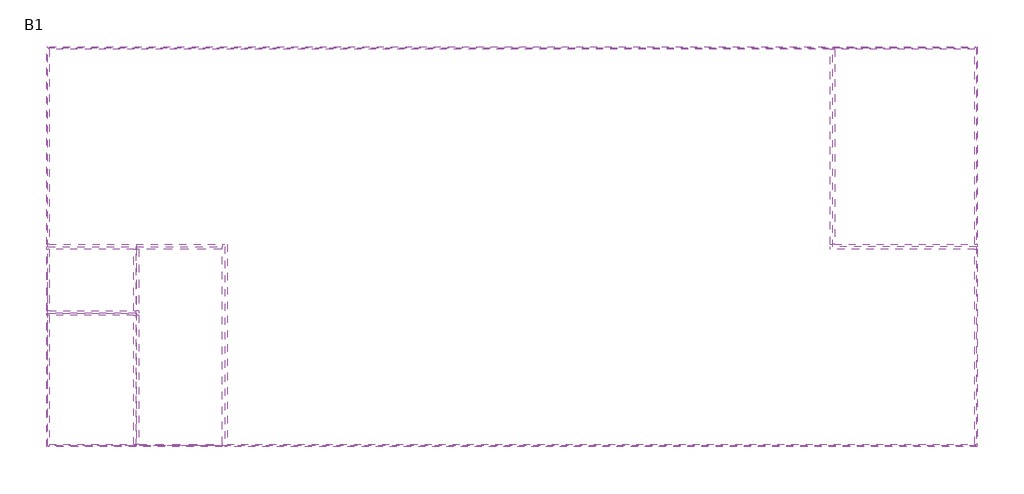
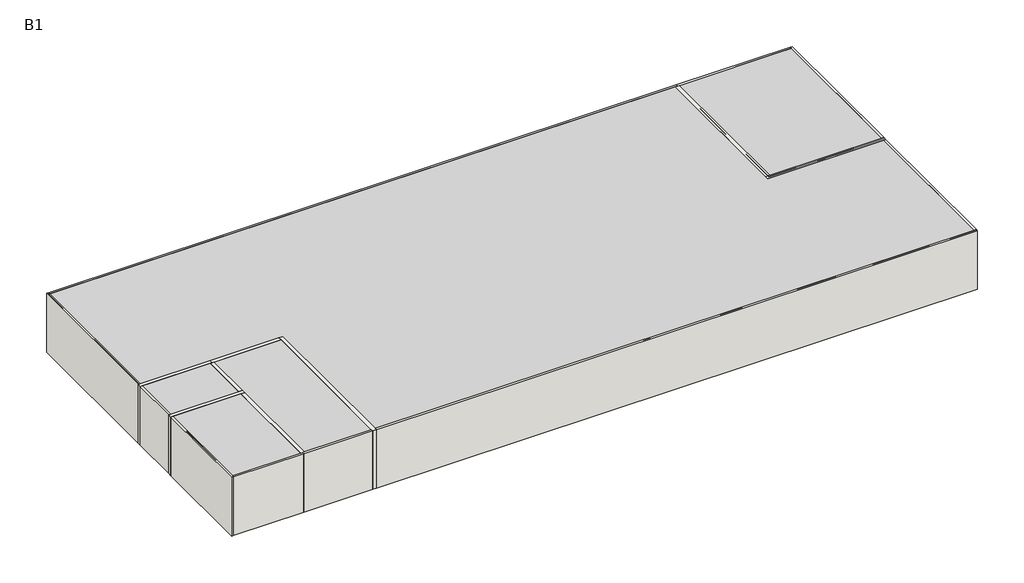
# One storey: 18 walls, 5 proxies.
"""IFC4 building model written with IfcOpenShell, lengths in millimetres."""

import ifcopenshell
import ifcopenshell.guid

model = None  # the IFC model being written
_history = None  # IfcOwnerHistory: only IFC2X3 demands one
_inside = {}  # id of a spatial element -> (the spatial element, [elements in it])
_under = {}  # id of a project, library or spatial element -> (it, [spatial elements below it])
_declared = {}  # id of a project -> (the project, [libraries it declares])
_typed = {}  # id of a type object -> (the type object, [elements of that type])
_made_of = {}  # id of a material, layer set ... -> (it, [elements and type objects made of it])


def new_model(schema):
    """Start an empty IFC model of exactly this schema.

    Asked for "IFC4X3", IfcOpenShell would pick the latest addendum, in which some entities
    have other attributes; the version numbers below select the first issue.
    IFC2X3 requires an IfcOwnerHistory on every rooted entity: one is made here for all.
    """
    global model, _history
    if schema == "IFC4X3":
        model = ifcopenshell.file(schema_version=(4, 3, 0, 0))
    else:
        model = ifcopenshell.file(schema=schema)
    _inside.clear()
    _under.clear()
    _declared.clear()
    _typed.clear()
    _made_of.clear()
    _history = None
    if model.schema == "IFC2X3":
        org = make("IfcOrganization", Name="unknown")
        user = make(
            "IfcPersonAndOrganization",
            ThePerson=make("IfcPerson", FamilyName="unknown"),
            TheOrganization=org,
        )
        app = make(
            "IfcApplication",
            ApplicationDeveloper=org,
            Version="unknown",
            ApplicationFullName="unknown",
            ApplicationIdentifier="unknown",
        )
        _history = make(
            "IfcOwnerHistory",
            OwningUser=user,
            OwningApplication=app,
            ChangeAction="ADDED",
            CreationDate=0,
        )
    return model


def make(cls, **values):
    """One entity of the class cls with the attributes given. An attribute that is None is left unset."""
    return model.create_entity(
        cls, **{name: value for name, value in values.items() if value is not None}
    )


def rooted(cls, **values):
    """An entity with a GlobalId (a new one), such as an element, a storey or a relation."""
    return make(cls, GlobalId=ifcopenshell.guid.new(), OwnerHistory=_history, **values)


def si_unit(unit_type, name, prefix=None):
    """IfcSIUnit, for example si_unit("LENGTHUNIT", "METRE", prefix="MILLI")."""
    return make("IfcSIUnit", UnitType=unit_type, Prefix=prefix, Name=name)


def assignment(units):
    """IfcUnitAssignment: the units of a project."""
    return None if units is None else make("IfcUnitAssignment", Units=units)


def point(xyz):
    """IfcCartesianPoint."""
    return None if xyz is None else make("IfcCartesianPoint", Coordinates=xyz)


def direction(xyz):
    """IfcDirection."""
    return None if xyz is None else make("IfcDirection", DirectionRatios=xyz)


def frame(location, z_axis=None, x_axis=None):
    """IfcAxis2Placement3D, a coordinate frame: its origin and axes. An axis left out is left unset."""
    return make(
        "IfcAxis2Placement3D",
        Location=point(location),
        Axis=direction(z_axis),
        RefDirection=direction(x_axis),
    )


def origin():
    """The frame at (0, 0, 0) with its axes left unset."""
    return frame((0.0, 0.0, 0.0))


def origin_with_axes():
    """The frame at (0, 0, 0) with the z axis (0, 0, 1) and the x axis (1, 0, 0) written out."""
    return frame((0.0, 0.0, 0.0), z_axis=(0.0, 0.0, 1.0), x_axis=(1.0, 0.0, 0.0))


def place(relative_to, where):
    """IfcLocalPlacement: puts the frame where relative to a parent placement (None: the world)."""
    return make(
        "IfcLocalPlacement", PlacementRelTo=relative_to, RelativePlacement=where
    )


def context(
    kind, dimensions, precision=None, world=None, true_north=None, identifier=None
):
    """IfcGeometricRepresentationContext, for example the 3D "Model" context."""
    return make(
        "IfcGeometricRepresentationContext",
        ContextIdentifier=identifier,
        ContextType=kind,
        CoordinateSpaceDimension=dimensions,
        Precision=precision,
        WorldCoordinateSystem=world,
        TrueNorth=true_north,
    )


def project(units=None, contexts=None):
    """IfcProject with its units and contexts."""
    return rooted(
        "IfcProject",
        Name="project",
        RepresentationContexts=contexts,
        UnitsInContext=assignment(units),
    )


def spatial(cls, under=None, at=None, **own):
    """A site, building, storey or space (cls), placed at a placement, below another one or the project."""
    s = rooted(cls, ObjectPlacement=at, **own)
    if under is not None:
        _under.setdefault(under.id(), (under, []))[1].append(s)
    return s


def polyline(points):
    """IfcPolyline through the points."""
    return make("IfcPolyline", Points=[point(p) for p in points])


def outline(outer, holes=None, kind="AREA"):
    """IfcArbitraryClosedProfileDef: a profile drawn as a closed curve; with holes, ...WithVoids."""
    if holes is None:
        return make("IfcArbitraryClosedProfileDef", ProfileType=kind, OuterCurve=outer)
    return make(
        "IfcArbitraryProfileDefWithVoids",
        ProfileType=kind,
        OuterCurve=outer,
        InnerCurves=holes,
    )


def extrude(swept, where, along, depth):
    """IfcExtrudedAreaSolid: the profile swept, set in the frame where, extruded along a direction by depth."""
    return make(
        "IfcExtrudedAreaSolid",
        SweptArea=swept,
        Position=where,
        ExtrudedDirection=direction(along),
        Depth=depth,
    )


def faces_of(points, faces, orient=None, outer=None):
    """IfcFace entities. A face is a list of loops; a loop is a list of indices into points, from 0.

    orient and outer hold one flag for each loop. By default every Orientation is true, the
    first loop of a face is its IfcFaceOuterBound and the others are IfcFaceBound.
    """
    made = []
    for i, loops in enumerate(faces):
        bounds = []
        for j, loop in enumerate(loops):
            is_outer = j == 0 if outer is None else outer[i][j]
            bounds.append(
                make(
                    "IfcFaceOuterBound" if is_outer else "IfcFaceBound",
                    Bound=make("IfcPolyLoop", Polygon=[points[k] for k in loop]),
                    Orientation=True if orient is None else orient[i][j],
                )
            )
        made.append(make("IfcFace", Bounds=bounds))
    return made


def faceted_brep(points, faces, orient=None, outer=None, voids=None):
    """IfcFacetedBrep: a solid bounded by flat faces; with voids (closed shells), ...WithVoids."""
    shared = [point(p) for p in points]
    hull = make("IfcClosedShell", CfsFaces=faces_of(shared, faces, orient, outer))
    if voids is None:
        return make("IfcFacetedBrep", Outer=hull)
    return make(
        "IfcFacetedBrepWithVoids",
        Outer=hull,
        Voids=[
            make(cls, CfsFaces=faces_of(shared, fs, o, b)) for cls, fs, o, b in voids
        ],
    )


def shape(context_of_items, identifier, shape_type, items):
    """IfcShapeRepresentation: the items that make up one representation, for example the "Body"."""
    return make(
        "IfcShapeRepresentation",
        ContextOfItems=context_of_items,
        RepresentationIdentifier=identifier,
        RepresentationType=shape_type,
        Items=items,
    )


def source(mapping_origin, context_of_items, identifier, shape_type, items):
    """IfcRepresentationMap: a shape defined once, which mapped items show again and again."""
    return make(
        "IfcRepresentationMap",
        MappingOrigin=mapping_origin,
        MappedRepresentation=shape(context_of_items, identifier, shape_type, items),
    )


def transform(
    local_origin,
    x_axis=None,
    y_axis=None,
    z_axis=None,
    scale=None,
    scale2=None,
    scale3=None,
    uniform=True,
):
    """IfcCartesianTransformationOperator3D, or its non-uniform kind. x_axis, y_axis, z_axis: its Axis1, 2, 3."""
    if uniform:
        return make(
            "IfcCartesianTransformationOperator3D",
            Axis1=direction(x_axis),
            Axis2=direction(y_axis),
            LocalOrigin=point(local_origin),
            Scale=scale,
            Axis3=direction(z_axis),
        )
    return make(
        "IfcCartesianTransformationOperator3DnonUniform",
        Axis1=direction(x_axis),
        Axis2=direction(y_axis),
        LocalOrigin=point(local_origin),
        Scale=scale,
        Axis3=direction(z_axis),
        Scale2=scale2,
        Scale3=scale3,
    )


def mapped(mapping_source, mapping_target):
    """IfcMappedItem: shows the shape of a source again, moved by a transform."""
    return make(
        "IfcMappedItem", MappingSource=mapping_source, MappingTarget=mapping_target
    )


def made_of(thing, what):
    """Note that an element or type object is made of a material, layer set ...; save() writes the relation."""
    if what is not None:
        _made_of.setdefault(what.id(), (what, []))[1].append(thing)
    return thing


def element(
    cls,
    number,
    at=None,
    inside=None,
    cuts=None,
    type_object=None,
    material=None,
    context=None,
    identifier="Body",
    shape_type=None,
    held_by="IfcProductDefinitionShape",
    body=None,
    shapes=None,
    **own,
):
    """One element of the class cls, such as IfcWall. Its Tag is "e" and its number.

    at: its placement. inside: the storey or other place that contains it. cuts: it is an
    opening in that element (IfcRelVoidsElement). A single representation is given by context,
    identifier, shape_type and body (its items); several are given by shapes. held_by: the class
    of the entity that holds the representations. save() writes the other relations.
    """
    e = rooted(cls, Tag="e%d" % number, ObjectPlacement=at, **own)
    if body is not None:
        shapes = [shape(context, identifier, shape_type, body)]
    if shapes is not None:
        e.Representation = make(held_by, Representations=shapes)
    if inside is not None:
        _inside.setdefault(inside.id(), (inside, []))[1].append(e)
    if cuts is not None:
        rooted(
            "IfcRelVoidsElement", RelatingBuildingElement=cuts, RelatedOpeningElement=e
        )
    if type_object is not None:
        _typed.setdefault(type_object.id(), (type_object, []))[1].append(e)
    return made_of(e, material)


def aggregate(whole, parts):
    """IfcRelAggregates: a whole, such as a stair, and the parts it consists of."""
    return rooted("IfcRelAggregates", RelatingObject=whole, RelatedObjects=parts)


def save(model, path):
    """Write the relations noted so far, then the file.

    IfcRelAggregates (storeys below a building ...), IfcRelContainedInSpatialStructure (elements
    in a storey), IfcRelDefinesByType, IfcRelAssociatesMaterial and IfcRelDeclares: one each for
    every whole, place, type object, material and project.
    """
    for whole, parts in _under.values():
        aggregate(whole, parts)
    for where, things in _inside.values():
        rooted(
            "IfcRelContainedInSpatialStructure",
            RelatedElements=things,
            RelatingStructure=where,
        )
    for kind, things in _typed.values():
        rooted("IfcRelDefinesByType", RelatedObjects=things, RelatingType=kind)
    for what, things in _made_of.values():
        rooted("IfcRelAssociatesMaterial", RelatedObjects=things, RelatingMaterial=what)
    for by, libraries in _declared.values():
        rooted("IfcRelDeclares", RelatingContext=by, RelatedDefinitions=libraries)
    model.write(path)


def generic_models_bb515c93(model_context):
    return source(origin(), model_context, "Body", "SweptSolid", [
        extrude(outline(polyline([(9000.0, 21000.0), (9000.0, -21000.0), (-9000.0, -21000.0), (-9000.0, 21000.0), (9000.0, 21000.0)])), origin_with_axes(), (0.0, 0.0, 1.0), 3500.0),
    ])


def generic_models_5926095e(model_context):
    return source(origin(), model_context, "Body", "SweptSolid", [
        extrude(outline(polyline([(3250.0, 4500.0), (3250.0, -4500.0), (-3250.0, -4500.0), (-3250.0, 4500.0), (3250.0, 4500.0)])), origin_with_axes(), (0.0, 0.0, 1.0), 3500.0),
    ])


def generic_models_0b067365(model_context):
    return source(origin(), model_context, "Body", "SweptSolid", [
        extrude(outline(polyline([(2000.0, 4500.0), (2000.0, -4500.0), (-2000.0, -4500.0), (-2000.0, 4500.0), (2000.0, 4500.0)])), origin_with_axes(), (0.0, 0.0, 1.0), 3500.0),
    ])


def generic_models_4c644d41(model_context):
    return source(origin(), model_context, "Body", "SweptSolid", [
        extrude(outline(polyline([(2000.0, 1500.0), (2000.0, -1500.0), (-2000.0, -1500.0), (-2000.0, 1500.0), (2000.0, 1500.0)])), origin_with_axes(), (0.0, 0.0, 1.0), 3500.0),
    ])


def generic_models_c89eb543(model_context):
    return source(origin(), model_context, "Body", "SweptSolid", [
        extrude(outline(polyline([(2000.0, 3000.0), (2000.0, -3000.0), (-2000.0, -3000.0), (-2000.0, 3000.0), (2000.0, 3000.0)])), origin_with_axes(), (0.0, 0.0, 1.0), 3500.0),
    ])


model = new_model("IFC4")

# Units and contexts
model_context = context("Model", 3, world=origin())
ifc_project = project(units=[si_unit("LENGTHUNIT", "METRE", prefix="MILLI")], contexts=[model_context])

# Site, building, storey
site = spatial("IfcSite", under=ifc_project)
building = spatial("IfcBuilding", under=site)
storey = spatial("IfcBuildingStorey", under=building, Name="B1", Elevation=-4000.0)

# Proxies
placement = place(None, origin())
generic_models_shape = generic_models_bb515c93(model_context)
element("IfcBuildingElementProxy", 1, Name="Space Planning Box_hec : Space Planning Box_hec", ObjectType="Space Planning Box_hec : Space Planning Box_hec", at=placement, inside=storey, context=model_context, shape_type="MappedRepresentation", body=[
    mapped(generic_models_shape, transform((66459.6521483, 172923.8614395, 0.0), x_axis=(0.0, -1.0, 0.0), y_axis=(1.0, 0.0, 0.0), z_axis=(0.0, 0.0, 1.0))),
])
generic_models_2_shape = generic_models_5926095e(model_context)
element("IfcBuildingElementProxy", 2, Name="Space Planning Box_hec : Space Planning Box_hec", ObjectType="Space Planning Box_hec : Space Planning Box_hec", at=placement, inside=storey, context=model_context, shape_type="MappedRepresentation", body=[
    mapped(generic_models_2_shape, transform((84209.6521483, 177423.8614395, 0.0), x_axis=(1.0, 0.0, 0.0), y_axis=(0.0, 1.0, 0.0), z_axis=(0.0, 0.0, 1.0))),
])
generic_models_3_shape = generic_models_0b067365(model_context)
element("IfcBuildingElementProxy", 3, Name="Space Planning Box_hec : Space Planning Box_hec", ObjectType="Space Planning Box_hec : Space Planning Box_hec", at=placement, inside=storey, context=model_context, shape_type="MappedRepresentation", body=[
    mapped(generic_models_3_shape, transform((51459.6521483, 168423.8614395, 0.0), x_axis=(1.0, 0.0, 0.0), y_axis=(0.0, 1.0, 0.0), z_axis=(0.0, 0.0, 1.0))),
])
generic_models_4_shape = generic_models_4c644d41(model_context)
element("IfcBuildingElementProxy", 4, Name="Space Planning Box_hec : Space Planning Box_hec", ObjectType="Space Planning Box_hec : Space Planning Box_hec", at=placement, inside=storey, context=model_context, shape_type="MappedRepresentation", body=[
    mapped(generic_models_4_shape, transform((47459.6521483, 171423.8614395, 0.0), x_axis=(1.0, 0.0, 0.0), y_axis=(0.0, 1.0, 0.0), z_axis=(0.0, 0.0, 1.0))),
])
generic_models_5_shape = generic_models_c89eb543(model_context)
element("IfcBuildingElementProxy", 5, Name="Space Planning Box_hec : Space Planning Box_hec", ObjectType="Space Planning Box_hec : Space Planning Box_hec", at=placement, inside=storey, context=model_context, shape_type="MappedRepresentation", body=[
    mapped(generic_models_5_shape, transform((47459.6521483, 166923.8614395, 0.0), x_axis=(1.0, 0.0, 0.0), y_axis=(0.0, 1.0, 0.0), z_axis=(0.0, 0.0, 1.0))),
])

# Walls
element("IfcWall", 6, ObjectType="WA211_Exterior-Cement Brick-90mm", at=placement, inside=storey, context=model_context, shape_type="Brep", body=[
    faceted_brep([(80959.6521483, 181866.8614395, 0.0), (81066.6521483, 181866.8614395, 0.0), (87402.6521483, 181866.8614395, 0.0), (87402.6521483, 181866.8614395, 3500.0), (81066.6521483, 181866.8614395, 3500.0), (80959.6521483, 181866.8614395, 3500.0), (80959.6521483, 181980.8614395, 0.0), (80959.6521483, 181980.8614395, 3500.0), (87402.6521483, 181980.8614395, 3500.0), (87402.6521483, 181980.8614395, 0.0)], [[[0, 1, 2, 3, 4, 5]], [[6, 7, 8, 9]], [[2, 1, 0, 6, 9]], [[5, 4, 3, 8, 7]], [[0, 5, 7, 6]], [[3, 2, 9, 8]]]),
])
element("IfcWall", 7, ObjectType="WA211_Exterior-Cement Brick-90mm", at=placement, inside=storey, context=model_context, shape_type="Brep", body=[
    faceted_brep([(87402.6521483, 181980.8614395, 0.0), (87402.6521483, 181866.8614395, 0.0), (87402.6521483, 173030.8614395, 0.0), (87402.6521483, 173030.8614395, 3500.0), (87402.6521483, 181866.8614395, 3500.0), (87402.6521483, 181980.8614395, 3500.0), (87516.6521483, 181980.8614395, 0.0), (87516.6521483, 181980.8614395, 3500.0), (87516.6521483, 173030.8614395, 3500.0), (87516.6521483, 173030.8614395, 0.0)], [[[0, 1, 2, 3, 4, 5]], [[6, 7, 8, 9]], [[2, 1, 0, 6, 9]], [[5, 4, 3, 8, 7]], [[0, 5, 7, 6]], [[3, 2, 9, 8]]]),
])
element("IfcWall", 8, ObjectType="WA211_Exterior-Cement Brick-90mm", at=placement, inside=storey, context=model_context, shape_type="Brep", body=[
    faceted_brep([(53352.6521483, 163980.8614395, 0.0), (49566.6521483, 163980.8614395, 0.0), (49459.6521483, 163980.8614395, 0.0), (49459.6521483, 163980.8614395, 3500.0), (49566.6521483, 163980.8614395, 3500.0), (53352.6521483, 163980.8614395, 3500.0), (53352.6521483, 163866.8614395, 0.0), (53352.6521483, 163866.8614395, 3500.0), (49459.6521483, 163866.8614395, 3500.0), (49459.6521483, 163866.8614395, 0.0)], [[[0, 1, 2, 3, 4, 5]], [[6, 7, 8, 9]], [[2, 1, 0, 6, 9]], [[3, 2, 9, 8]], [[5, 4, 3, 8, 7]], [[0, 5, 7, 6]]]),
])
element("IfcWall", 9, ObjectType="WA211_Exterior-Cement Brick-90mm", at=placement, inside=storey, context=model_context, shape_type="Brep", body=[
    faceted_brep([(45516.6521483, 173030.8614395, 0.0), (45516.6521483, 181866.8614395, 0.0), (45516.6521483, 181980.8614395, 0.0), (45516.6521483, 181980.8614395, 3500.0), (45516.6521483, 181866.8614395, 3500.0), (45516.6521483, 173030.8614395, 3500.0), (45402.6521483, 173030.8614395, 0.0), (45402.6521483, 173030.8614395, 3500.0), (45402.6521483, 181980.8614395, 3500.0), (45402.6521483, 181980.8614395, 0.0)], [[[0, 1, 2, 3, 4, 5]], [[6, 7, 8, 9]], [[2, 1, 0, 6, 9]], [[5, 4, 3, 8, 7]], [[3, 2, 9, 8]], [[0, 5, 7, 6]]]),
])
element("IfcWall", 10, ObjectType="WA211_Exterior-Cement Brick-90mm", at=placement, inside=storey, context=model_context, shape_type="Brep", body=[
    faceted_brep([(87516.6521483, 163980.8614395, 0.0), (87402.6521483, 163980.8614395, 0.0), (53566.6521483, 163980.8614395, 0.0), (53566.6521483, 163980.8614395, 3500.0), (87402.6521483, 163980.8614395, 3500.0), (87516.6521483, 163980.8614395, 3500.0), (87516.6521483, 163866.8614395, 0.0), (87516.6521483, 163866.8614395, 3500.0), (53566.6521483, 163866.8614395, 3500.0), (53566.6521483, 163866.8614395, 0.0)], [[[0, 1, 2, 3, 4, 5]], [[6, 7, 8, 9]], [[2, 1, 0, 6, 9]], [[5, 4, 3, 8, 7]], [[0, 5, 7, 6]], [[3, 2, 9, 8]]]),
])
element("IfcWall", 11, ObjectType="WA211_Exterior-Cement Brick-90mm", at=placement, inside=storey, context=model_context, shape_type="SweptSolid", body=[
    extrude(outline(polyline([(87402.6521483, 163980.8614395), (87402.6521483, 172816.8614395), (87516.6521483, 172816.8614395), (87516.6521483, 163980.8614395), (87402.6521483, 163980.8614395)])), origin_with_axes(), (0.0, 0.0, 1.0), 3500.0),
])
element("IfcWall", 12, ObjectType="WA211_Exterior-Cement Brick-90mm", at=placement, inside=storey, context=model_context, shape_type="Brep", body=[
    faceted_brep([(45516.6521483, 181866.8614395, 0.0), (80852.6521483, 181866.8614395, 0.0), (80959.6521483, 181866.8614395, 0.0), (80959.6521483, 181866.8614395, 3500.0), (80852.6521483, 181866.8614395, 3500.0), (45516.6521483, 181866.8614395, 3500.0), (45516.6521483, 181980.8614395, 0.0), (45516.6521483, 181980.8614395, 3500.0), (80959.6521483, 181980.8614395, 3500.0), (80959.6521483, 181980.8614395, 0.0)], [[[0, 1, 2, 3, 4, 5]], [[6, 7, 8, 9]], [[2, 1, 0, 6, 9]], [[3, 2, 9, 8]], [[5, 4, 3, 8, 7]], [[0, 5, 7, 6]]]),
])
element("IfcWall", 13, ObjectType="WA211_Exterior-Cement Brick-90mm", at=placement, inside=storey, context=model_context, shape_type="Brep", body=[
    faceted_brep([(49459.6521483, 163980.8614395, 0.0), (49352.6521483, 163980.8614395, 0.0), (45516.6521483, 163980.8614395, 0.0), (45516.6521483, 163980.8614395, 3500.0), (49352.6521483, 163980.8614395, 3500.0), (49459.6521483, 163980.8614395, 3500.0), (49459.6521483, 163866.8614395, 0.0), (49459.6521483, 163866.8614395, 3500.0), (45516.6521483, 163866.8614395, 3500.0), (45516.6521483, 163866.8614395, 0.0)], [[[0, 1, 2, 3, 4, 5]], [[6, 7, 8, 9]], [[2, 1, 0, 6, 9]], [[5, 4, 3, 8, 7]], [[0, 5, 7, 6]], [[3, 2, 9, 8]]]),
])
element("IfcWall", 14, ObjectType="WA211_Exterior-Cement Brick-90mm", at=placement, inside=storey, context=model_context, shape_type="Brep", body=[
    faceted_brep([(45516.6521483, 163866.8614395, 0.0), (45516.6521483, 163980.8614395, 0.0), (45516.6521483, 169816.8614395, 0.0), (45516.6521483, 169816.8614395, 3500.0), (45516.6521483, 163980.8614395, 3500.0), (45516.6521483, 163866.8614395, 3500.0), (45402.6521483, 163866.8614395, 0.0), (45402.6521483, 163866.8614395, 3500.0), (45402.6521483, 169816.8614395, 3500.0), (45402.6521483, 169816.8614395, 0.0)], [[[0, 1, 2, 3, 4, 5]], [[6, 7, 8, 9]], [[2, 1, 0, 6, 9]], [[5, 4, 3, 8, 7]], [[0, 5, 7, 6]], [[3, 2, 9, 8]]]),
])
element("IfcWall", 15, ObjectType="WA211_Exterior-Cement Brick-90mm", at=placement, inside=storey, context=model_context, shape_type="SweptSolid", body=[
    extrude(outline(polyline([(45516.6521483, 172816.8614395), (45516.6521483, 170030.8614395), (45402.6521483, 170030.8614395), (45402.6521483, 172816.8614395), (45516.6521483, 172816.8614395)])), origin_with_axes(), (0.0, 0.0, 1.0), 3500.0),
])
element("IfcWall", 16, ObjectType="WA221_Interior-Cement Block-190mm", at=placement, inside=storey, context=model_context, shape_type="Brep", body=[
    faceted_brep([(80852.6521483, 181866.8614395, 0.0), (80852.6521483, 173030.8614395, 0.0), (80852.6521483, 173030.8614395, 3500.0), (80852.6521483, 181866.8614395, 3500.0), (81066.6521483, 181866.8614395, 0.0), (81066.6521483, 181866.8614395, 3500.0), (81066.6521483, 173030.8614395, 3500.0), (81066.6521483, 173030.8614395, 0.0), (80959.6521483, 181866.8614395, 0.0), (80959.6521483, 181866.8614395, 3500.0)], [[[0, 1, 2, 3]], [[4, 5, 6, 7]], [[1, 0, 8, 4, 7]], [[3, 2, 6, 5, 9]], [[0, 3, 9, 5, 4, 8]], [[2, 1, 7, 6]]]),
])
element("IfcWall", 17, ObjectType="WA221_Interior-Cement Block-190mm", at=placement, inside=storey, context=model_context, shape_type="Brep", body=[
    faceted_brep([(87516.6521483, 173030.8614395, 0.0), (87402.6521483, 173030.8614395, 0.0), (81066.6521483, 173030.8614395, 0.0), (80852.6521483, 173030.8614395, 0.0), (80852.6521483, 173030.8614395, 3500.0), (81066.6521483, 173030.8614395, 3500.0), (87402.6521483, 173030.8614395, 3500.0), (87516.6521483, 173030.8614395, 3500.0), (87516.6521483, 172816.8614395, 0.0), (87516.6521483, 172816.8614395, 3500.0), (87402.6521483, 172816.8614395, 3500.0), (80852.6521483, 172816.8614395, 3500.0), (80852.6521483, 172816.8614395, 0.0), (87402.6521483, 172816.8614395, 0.0)], [[[0, 1, 2, 3, 4, 5, 6, 7]], [[8, 9, 10, 11, 12, 13]], [[3, 2, 1, 0, 8, 13, 12]], [[7, 6, 5, 4, 11, 10, 9]], [[4, 3, 12, 11]], [[0, 7, 9, 8]]]),
])
element("IfcWall", 18, ObjectType="WA221_Interior-Cement Block-190mm", at=placement, inside=storey, context=model_context, shape_type="Brep", body=[
    faceted_brep([(53566.6521483, 163866.8614395, 0.0), (53566.6521483, 163980.8614395, 0.0), (53566.6521483, 173030.8614395, 0.0), (53566.6521483, 173030.8614395, 3500.0), (53566.6521483, 163980.8614395, 3500.0), (53566.6521483, 163866.8614395, 3500.0), (53352.6521483, 163866.8614395, 0.0), (53352.6521483, 163866.8614395, 3500.0), (53352.6521483, 163980.8614395, 3500.0), (53352.6521483, 172816.8614395, 3500.0), (53352.6521483, 173030.8614395, 3500.0), (53352.6521483, 173030.8614395, 0.0), (53352.6521483, 172816.8614395, 0.0), (53352.6521483, 163980.8614395, 0.0)], [[[0, 1, 2, 3, 4, 5]], [[6, 7, 8, 9, 10, 11, 12, 13]], [[2, 1, 0, 6, 13, 12, 11]], [[5, 4, 3, 10, 9, 8, 7]], [[3, 2, 11, 10]], [[0, 5, 7, 6]]]),
])
element("IfcWall", 19, ObjectType="WA221_Interior-Cement Block-190mm", at=placement, inside=storey, context=model_context, shape_type="Brep", body=[
    faceted_brep([(49459.6521483, 172816.8614395, 0.0), (49566.6521483, 172816.8614395, 0.0), (53352.6521483, 172816.8614395, 0.0), (53352.6521483, 172816.8614395, 3500.0), (49566.6521483, 172816.8614395, 3500.0), (49459.6521483, 172816.8614395, 3500.0), (49459.6521483, 173030.8614395, 0.0), (49459.6521483, 173030.8614395, 3500.0), (53352.6521483, 173030.8614395, 3500.0), (53352.6521483, 173030.8614395, 0.0)], [[[0, 1, 2, 3, 4, 5]], [[6, 7, 8, 9]], [[2, 1, 0, 6, 9]], [[5, 4, 3, 8, 7]], [[0, 5, 7, 6]], [[3, 2, 9, 8]]]),
])
element("IfcWall", 20, ObjectType="WA221_Interior-Cement Block-190mm", at=placement, inside=storey, context=model_context, shape_type="Brep", body=[
    faceted_brep([(49352.6521483, 169816.8614395, 0.0), (49352.6521483, 163980.8614395, 0.0), (49352.6521483, 163980.8614395, 3500.0), (49352.6521483, 169816.8614395, 3500.0), (49566.6521483, 169816.8614395, 0.0), (49566.6521483, 169816.8614395, 3500.0), (49566.6521483, 163980.8614395, 3500.0), (49566.6521483, 163980.8614395, 0.0), (49459.6521483, 163980.8614395, 0.0), (49459.6521483, 163980.8614395, 3500.0)], [[[0, 1, 2, 3]], [[4, 5, 6, 7]], [[1, 0, 4, 7, 8]], [[3, 2, 9, 6, 5]], [[2, 1, 8, 7, 6, 9]], [[0, 3, 5, 4]]]),
])
element("IfcWall", 21, ObjectType="WA221_Interior-Cement Block-190mm", at=placement, inside=storey, context=model_context, shape_type="Brep", body=[
    faceted_brep([(49352.6521483, 172816.8614395, 0.0), (49352.6521483, 170030.8614395, 0.0), (49352.6521483, 170030.8614395, 3500.0), (49352.6521483, 172816.8614395, 3500.0), (49566.6521483, 172816.8614395, 0.0), (49566.6521483, 172816.8614395, 3500.0), (49566.6521483, 170030.8614395, 3500.0), (49566.6521483, 170030.8614395, 0.0), (49459.6521483, 172816.8614395, 0.0), (49459.6521483, 172816.8614395, 3500.0)], [[[0, 1, 2, 3]], [[4, 5, 6, 7]], [[1, 0, 8, 4, 7]], [[3, 2, 6, 5, 9]], [[0, 3, 9, 5, 4, 8]], [[2, 1, 7, 6]]]),
])
element("IfcWall", 22, ObjectType="WA221_Interior-Cement Block-190mm", at=placement, inside=storey, context=model_context, shape_type="Brep", body=[
    faceted_brep([(49459.6521483, 173030.8614395, 0.0), (45516.6521483, 173030.8614395, 0.0), (45402.6521483, 173030.8614395, 0.0), (45402.6521483, 173030.8614395, 3500.0), (45516.6521483, 173030.8614395, 3500.0), (49459.6521483, 173030.8614395, 3500.0), (49459.6521483, 172816.8614395, 0.0), (49459.6521483, 172816.8614395, 3500.0), (49352.6521483, 172816.8614395, 3500.0), (45516.6521483, 172816.8614395, 3500.0), (45402.6521483, 172816.8614395, 3500.0), (45402.6521483, 172816.8614395, 0.0), (45516.6521483, 172816.8614395, 0.0), (49352.6521483, 172816.8614395, 0.0)], [[[0, 1, 2, 3, 4, 5]], [[6, 7, 8, 9, 10, 11, 12, 13]], [[2, 1, 0, 6, 13, 12, 11]], [[5, 4, 3, 10, 9, 8, 7]], [[0, 5, 7, 6]], [[3, 2, 11, 10]]]),
])
element("IfcWall", 23, ObjectType="WA221_Interior-Cement Block-190mm", at=placement, inside=storey, context=model_context, shape_type="Brep", body=[
    faceted_brep([(49566.6521483, 170030.8614395, 0.0), (49352.6521483, 170030.8614395, 0.0), (45516.6521483, 170030.8614395, 0.0), (45402.6521483, 170030.8614395, 0.0), (45402.6521483, 170030.8614395, 3500.0), (45516.6521483, 170030.8614395, 3500.0), (49352.6521483, 170030.8614395, 3500.0), (49566.6521483, 170030.8614395, 3500.0), (49566.6521483, 169816.8614395, 0.0), (49566.6521483, 169816.8614395, 3500.0), (49352.6521483, 169816.8614395, 3500.0), (45516.6521483, 169816.8614395, 3500.0), (45402.6521483, 169816.8614395, 3500.0), (45402.6521483, 169816.8614395, 0.0), (45516.6521483, 169816.8614395, 0.0), (49352.6521483, 169816.8614395, 0.0)], [[[0, 1, 2, 3, 4, 5, 6, 7]], [[8, 9, 10, 11, 12, 13, 14, 15]], [[3, 2, 1, 0, 8, 15, 14, 13]], [[7, 6, 5, 4, 12, 11, 10, 9]], [[0, 7, 9, 8]], [[4, 3, 13, 12]]]),
])

save(model, "model.ifc")

# Revit data of these elements
# Project information
#   Building Name = "MAIN GATE SECURITY BUILDING"
#   Project Status = "Project Status"
#   Client Name = "현대엔지니어링"
#   Project Address = "서울시 종로구 율곡로 75(계동)"
#   Project Name = "Therma Visayas Energy Project"
#   Project Number = "-"
# Grids (mm)
#   "1": line (45459.652, 190234.526) -> (45459.652, 152139.384)
#   "2": line (53459.652, 190234.526) -> (53459.652, 152139.384)
#   "3": line (61459.652, 190234.526) -> (61459.652, 152139.384)
#   "4": line (69459.652, 190234.526) -> (69459.652, 152139.384)
#   "5": line (77459.652, 190234.526) -> (77459.652, 152139.384)
#   "6": line (87459.652, 190234.526) -> (87459.652, 152139.384)
#   "C": line (39389.066, 181923.861) -> (102402.798, 181923.861)
#   "B": line (39389.066, 172923.861) -> (102402.798, 172923.861)
#   "A": line (39389.066, 163923.861) -> (102402.798, 163923.861)
# Type "Space Planning Box_hec : Space Planning Box_hec"
#   Type Comments = "..."
#   Room Name [instance default] = "?"
#   Interior Finish [instance default] = ""
#   Exterior Finish [instance default] = ""
#   Department [instance default] = ""
#   Assembly Code = "..."
#   ceiling height [instance default] = 0
#   Width [instance default] = 1524 mm
#   Program Area [instance default] = 0.00 m²
#   Length [instance default] = 1524 mm
#   Height [instance default] = 1524 mm
#   Area [instance default] = 2.32258 m²
#   Fill Color [instance default] = Cyan
#   Default Elevation = 0
# Type "WA211_Exterior-Cement Brick-90mm"
#   Type Comments = ""
#   Layers, outside or top first: 0 mm "A04AL081-00001_Skirt_Acrylic Emulsion Paint" (function 100); 0 mm "A04AL077-00001_Ext Wall Painting_Acrylic Emulsion Paint" (function 100); 12 mm "A04AS164-00001_Plastering_Ext" (function 4); 90 mm "A04AK073-00001_Concrete Brick_0.5B" (function 1); 12 mm "A04AS164-00002_Plastering_Int" (function 5); 0 mm "A04AL078-00002_Int Wall Painting_Water Emulsion Paint" (function 100); 0 mm "A04AL081-00001_Skirt_Acrylic Emulsion Paint" (function 100)
# Type "WA221_Interior-Cement Block-190mm"
#   Type Comments = ""
#   Layers, outside or top first: 0 mm "A04AL081-00001_Skirt_Acrylic Emulsion Paint" (function 100); 0 mm "A04AL078-00002_Int Wall Painting_Water Emulsion Paint" (function 100); 12 mm "A04AS164-00002_Plastering_Int" (function 2); 190 mm "A04AK069-00002_Reinforced Concrete Block_THK 100-200mm" (function 1); 12 mm "A04AS164-00002_Plastering_Int" (function 2); 0 mm "A04AL078-00002_Int Wall Painting_Water Emulsion Paint" (function 100); 0 mm "A04AL081-00001_Skirt_Acrylic Emulsion Paint" (function 100)
# Element 1 (IfcBuildingElementProxy, "Space Planning Box_hec : Space Planning Box_hec")
#   Room Name = "Cable Room"
#   Interior Finish = "IW5..IW2..N/A,,WK1..N/A,,FL1..N/A,,CL1..N/A"
#   Exterior Finish = "N/A..N/A,,EW1..EW2..N/A"
#   Department = "EL"
#   ceiling height = 0
#   Width = 18000 mm
#   Program Area = 720.00 m²
#   Length = 42000 mm
#   Height = 3500 mm
#   Area = 756.00 m²
#   Fill Color = Orange
#   Phase Created = New Construction
#   Materials on its faces: "Orange"
# Element 2 (IfcBuildingElementProxy, "Space Planning Box_hec : Space Planning Box_hec")
#   Room Name = "Battery Room"
#   Interior Finish = "IW2..N/A..N/A,,N/A..N/A,,FL7..N/A,,CL2..N/A"
#   Exterior Finish = "N/A..N/A,,EW2..N/A..N/A"
#   Department = "EL"
#   ceiling height = 0
#   Width = 6500 mm
#   Program Area = 58.50 m²
#   Length = 9000 mm
#   Height = 3500 mm
#   Area = 58.50 m²
#   Fill Color = Orange
#   Phase Created = New Construction
#   Materials on its faces: "Orange"
# Element 3 (IfcBuildingElementProxy, "Space Planning Box_hec : Space Planning Box_hec")
#   Room Name = "Lobby"
#   Interior Finish = "IW5..N/A..N/A,,WK3..N/A,,FL2..N/A,,N/A..N/A"
#   Exterior Finish = "N/A..N/A,,EW2..N/A..N/A"
#   Department = "AR"
#   ceiling height = 0
#   Width = 4000 mm
#   Program Area = 0.00 m²
#   Length = 9000 mm
#   Height = 3500 mm
#   Area = 36.00 m²
#   Fill Color = Cyan
#   Phase Created = New Construction
#   Materials on its faces: "Cyan"
# Element 4 (IfcBuildingElementProxy, "Space Planning Box_hec : Space Planning Box_hec")
#   Room Name = "Elevator"
#   Interior Finish = "N/A..N/A..N/A,,N/A..N/A,,,,CL3..N/A"
#   Exterior Finish = "N/A..N/A,,EW2..N/A..N/A"
#   Department = "AR"
#   ceiling height = 0
#   Width = 4000 mm
#   Program Area = 0.00 m²
#   Length = 3000 mm
#   Height = 3500 mm
#   Area = 12.00 m²
#   Fill Color = Cyan
#   Phase Created = New Construction
#   Materials on its faces: "Cyan"
# Element 5 (IfcBuildingElementProxy, "Space Planning Box_hec : Space Planning Box_hec")
#   Room Name = "Stairway"
#   Interior Finish = "IW5..N/A..N/A,,WK3..N/A,,FL2..N/A,,CL1..N/A"
#   Exterior Finish = "N/A..N/A,,EW2..N/A..N/A"
#   Department = "PATHV1"
#   ceiling height = 0
#   Width = 4000 mm
#   Program Area = 36.00 m²
#   Length = 6000 mm
#   Height = 3500 mm
#   Area = 24.00 m²
#   Fill Color = Green
#   Phase Created = New Construction
#   Materials on its faces: "Green"
# Elements 6, 8, 11, 12, 13, 15 (IfcWall, "WA211_Exterior-Cement Brick-90mm")
#   Top Offset = 0 mm
#   Base Offset = 0 mm
#   Unconnected Height = 3500 mm
#   wall height = 3500 mm
#   Phase Created = New Construction
#   Base Constraint = GF
#   Materials on its faces: "Default Wall", "A04AS164-00002_Plastering_Int", "A04AS164-00001_Plastering_Ext"
# Elements 7, 9, 10, 14 (IfcWall, "WA211_Exterior-Cement Brick-90mm")
#   Top Offset = 0 mm
#   Base Offset = 0 mm
#   Unconnected Height = 3500 mm
#   wall height = 3500 mm
#   Phase Created = New Construction
#   Base Constraint = GF
#   Materials on its faces: "Default Wall", "A04AS164-00001_Plastering_Ext", "A04AS164-00002_Plastering_Int"
# Elements 16, 19, 20, 21 (IfcWall, "WA221_Interior-Cement Block-190mm")
#   Top Offset = 0 mm
#   Base Offset = 0 mm
#   Unconnected Height = 3500 mm
#   wall height = 3500 mm
#   Phase Created = New Construction
#   Base Constraint = GF
#   Materials on its faces: "Default Wall", "A04AS164-00002_Plastering_Int"
# Elements 17, 18, 23 (IfcWall, "WA221_Interior-Cement Block-190mm")
#   Top Offset = 0 mm
#   Base Offset = 0 mm
#   Unconnected Height = 3500 mm
#   wall height = 3500 mm
#   Phase Created = New Construction
#   Base Constraint = GF
#   Materials on its faces: "A04AS164-00002_Plastering_Int", "Default Wall", "A04AS164-00001_Plastering_Ext"
# Element 22 (IfcWall, "WA221_Interior-Cement Block-190mm")
#   Top Offset = 0 mm
#   Base Offset = 0 mm
#   Unconnected Height = 3500 mm
#   wall height = 3500 mm
#   Phase Created = New Construction
#   Base Constraint = GF
#   Materials on its faces: "Default Wall", "A04AS164-00002_Plastering_Int", "A04AS164-00001_Plastering_Ext"
# Materials
#   "Cyan": class "Generic", colour RGB 0 255 255, transparency 0.2, Cost = 0
#   "A04AL081-00001_Skirt_Acrylic Emulsion Paint": class "Finish", colour RGB 128 128 64, transparency 0, Description = "Plastic", W00) Work Master Code = "A04AL081-00001", W01) Work Master_Lv1 = "Finishing Work", W02) Work Master_Lv2 = "Painting Work", W03) Work Master_Spec.1 = "Skirt Painting", W04) Work Master_Spec.2 = "Acrylic Emulsion Paint", W05) Work Master_Spec.3 = "100mm≤H<150mm", Cost = 0
#   "A04AL077-00001_Ext Wall Painting_Acrylic Emulsion Paint": class "Finish", colour RGB 128 128 64, transparency 0, Description = "Plastic", W00) Work Master Code = "A04AL077-00001", W01) Work Master_Lv1 = "Finishing Work", W02) Work Master_Lv2 = "Painting Work", W03) Work Master_Spec.1 = "External Wall Painting", W04) Work Master_Spec.2 = "Acrylic Emulsion Paint", Cost = 0
#   "A04AS164-00001_Plastering_Ext": class "Concrete", colour RGB 183 186 184, transparency 0, W00) Work Master Code = "A04AS164-00001", W01) Work Master_Lv1 = "Finishing Work", W02) Work Master_Lv2 = "Plastering Work", W03) Work Master_Spec.1 = "Plastering", W04) Work Master_Spec.2 = "for External Masonry Wall", Cost = 0
#   "A04AK073-00001_Concrete Brick_0.5B": class "Concrete", colour RGB 180 180 180, transparency 0, Description = "Conc. Block", W00) Work Master Code = "A04AK073-00001", W01) Work Master_Lv1 = "Finishing Work", W02) Work Master_Lv2 = "Masonry Work", W03) Work Master_Spec.1 = "Concrete Brick", W04) Work Master_Spec.2 = "[0.5B] w/ All Reinf.(Lath, Steel Tie, Anchor Bar, Mortar, ETC.), Filler, Sealant, Lintel/Sill for Opening, ETC.", Cost = 0
#   "A04AS164-00002_Plastering_Int": class "Concrete", colour RGB 183 186 184, transparency 0, Description = "LATEX PAINT ON THK.15 CEMENT PLASTER", W00) Work Master Code = "A04AS164-00002", W01) Work Master_Lv1 = "Finishing Work", W02) Work Master_Lv2 = "Plastering Work", W03) Work Master_Spec.1 = "Plastering", W04) Work Master_Spec.2 = "for Internal Masonry Wall", Cost = 0
#   "A04AL078-00002_Int Wall Painting_Water Emulsion Paint": class "Finish", colour RGB 128 128 64, transparency 0, Description = "Plastic", W00) Work Master Code = "A04AL078-00002", W01) Work Master_Lv1 = "Finishing Work", W02) Work Master_Lv2 = "Painting Work", W03) Work Master_Spec.1 = "Internal Wall Painting", W04) Work Master_Spec.2 = "Water Emulsion Paint", Cost = 0
#   "A04AK069-00002_Reinforced Concrete Block_THK 100-200mm": class "Concrete", colour RGB 180 180 180, transparency 0, Description = "Conc. Block", W00) Work Master Code = "A04AK069-00002", W01) Work Master_Lv1 = "Finishing Work", W02) Work Master_Lv2 = "Masonry Work", W03) Work Master_Spec.1 = "Reinforced Concrete Block", W04) Work Master_Spec.2 = "w/ All Reinf.(Lath, Steel Tie, Anchor Bar, Mortar, ETC.), Filler, Sealant, Lintel/Sill for Opening, ETC.", W05) Work Master_Spec.3 = "100mm<THK≤200mm", Cost = 0
#   "Orange": class "Generic", colour RGB 255 165 0, transparency 0.2, Cost = 0
#   "Green": class "Generic", colour RGB 0 128 0, transparency 0.2, Cost = 0
#   "Default Wall": class "Miscellaneous", colour RGB 80 80 80, transparency 0
# Room at (84209.652, 177423.861) mm, phase "New Construction", upper offset 3500 mm, lower offset 0 mm
#   Department = "EL"
#   Base Finish = ""
#   Ceiling Finish = "CL2"
#   Wall Finish = "IW2"
#   Floor Finish = "FL7"
#   Number = "0.0"
#   Name = "Battery Room"
#   Interior Finish = "IW2..N/A..N/A,,N/A..N/A,,FL7..N/A,,CL2..N/A"
#   Exterior Finish = "N/A..N/A,,EW2..N/A..N/A"
# Room at (51459.652, 168423.861) mm, phase "New Construction", upper offset 3500 mm, lower offset 0 mm
#   Department = "AR"
#   Base Finish = "WK3"
#   Ceiling Finish = ""
#   Wall Finish = "IW5"
#   Floor Finish = "FL2"
#   Number = "0.1"
#   Name = "Lobby"
#   Interior Finish = "IW5..N/A..N/A,,WK3..N/A,,FL2..N/A,,N/A..N/A"
#   Exterior Finish = "N/A..N/A,,EW2..N/A..N/A"
# Room at (66459.652, 172923.861) mm, phase "New Construction", upper offset 3500 mm, lower offset 0 mm
#   Department = "EL"
#   Base Finish = "WK1"
#   Ceiling Finish = "CL1"
#   Wall Finish = "IW5,IW2"
#   Floor Finish = "FL1"
#   Number = "0.2"
#   Name = "Cable Room"
#   Interior Finish = "IW5..IW2..N/A,,WK1..N/A,,FL1..N/A,,CL1..N/A"
#   Exterior Finish = "N/A..N/A,,EW1..EW2..N/A"
# Room at (47459.652, 166923.861) mm, phase "New Construction", upper offset 3500 mm, lower offset 0 mm
#   Department = "PATHV1"
#   Base Finish = "WK3"
#   Ceiling Finish = "CL1"
#   Wall Finish = "IW5"
#   Floor Finish = "FL2"
#   Number = "0.3"
#   Name = "Stairway"
#   Interior Finish = "IW5..N/A..N/A,,WK3..N/A,,FL2..N/A,,CL1..N/A"
#   Exterior Finish = "N/A..N/A,,EW2..N/A..N/A"
# Room at (47459.652, 171423.861) mm, phase "New Construction", upper offset 3500 mm, lower offset 0 mm
#   Department = "AR"
#   Base Finish = ""
#   Ceiling Finish = "CL3"
#   Wall Finish = ""
#   Floor Finish = ""
#   Number = "0.4"
#   Name = "Elevator"
#   Interior Finish = "N/A..N/A..N/A,,N/A..N/A,,,,CL3..N/A"
#   Exterior Finish = "N/A..N/A,,EW2..N/A..N/A"
